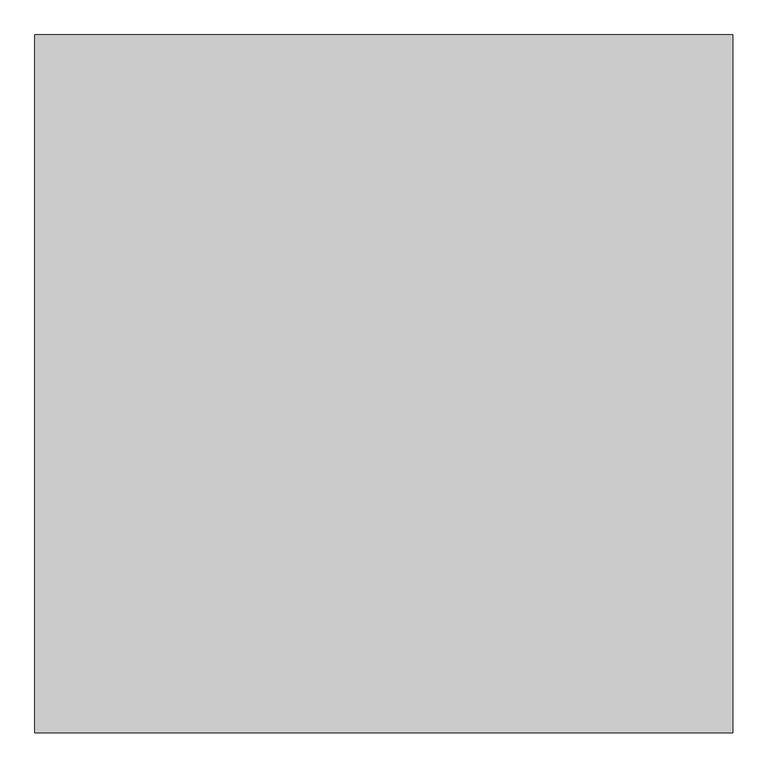
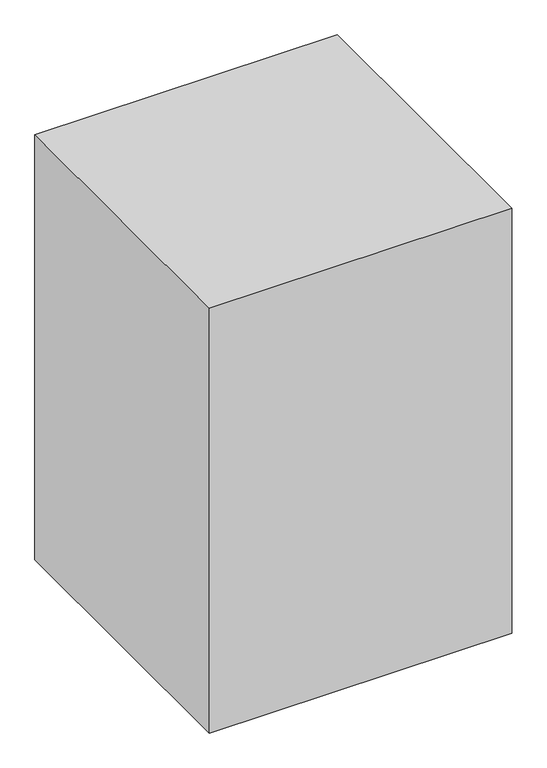
"""IFC4 building model written with IfcOpenShell, lengths in millimetres: proxy geometry, Space Planning Box_hec : Space Planning Box_hec."""

import ifcopenshell
import ifcopenshell.guid

model = None  # the IFC model being written
_history = None  # IfcOwnerHistory: only IFC2X3 demands one
_inside = {}  # id of a spatial element -> (the spatial element, [elements in it])
_under = {}  # id of a project, library or spatial element -> (it, [spatial elements below it])
_declared = {}  # id of a project -> (the project, [libraries it declares])
_typed = {}  # id of a type object -> (the type object, [elements of that type])
_made_of = {}  # id of a material, layer set ... -> (it, [elements and type objects made of it])


def new_model(schema):
    """Start an empty IFC model of exactly this schema.

    Asked for "IFC4X3", IfcOpenShell would pick the latest addendum, in which some entities
    have other attributes; the version numbers below select the first issue.
    IFC2X3 requires an IfcOwnerHistory on every rooted entity: one is made here for all.
    """
    global model, _history
    if schema == "IFC4X3":
        model = ifcopenshell.file(schema_version=(4, 3, 0, 0))
    else:
        model = ifcopenshell.file(schema=schema)
    _inside.clear()
    _under.clear()
    _declared.clear()
    _typed.clear()
    _made_of.clear()
    _history = None
    if model.schema == "IFC2X3":
        org = make("IfcOrganization", Name="unknown")
        user = make(
            "IfcPersonAndOrganization",
            ThePerson=make("IfcPerson", FamilyName="unknown"),
            TheOrganization=org,
        )
        app = make(
            "IfcApplication",
            ApplicationDeveloper=org,
            Version="unknown",
            ApplicationFullName="unknown",
            ApplicationIdentifier="unknown",
        )
        _history = make(
            "IfcOwnerHistory",
            OwningUser=user,
            OwningApplication=app,
            ChangeAction="ADDED",
            CreationDate=0,
        )
    return model


def make(cls, **values):
    """One entity of the class cls with the attributes given. An attribute that is None is left unset."""
    return model.create_entity(
        cls, **{name: value for name, value in values.items() if value is not None}
    )


def rooted(cls, **values):
    """An entity with a GlobalId (a new one), such as an element, a storey or a relation."""
    return make(cls, GlobalId=ifcopenshell.guid.new(), OwnerHistory=_history, **values)


def si_unit(unit_type, name, prefix=None):
    """IfcSIUnit, for example si_unit("LENGTHUNIT", "METRE", prefix="MILLI")."""
    return make("IfcSIUnit", UnitType=unit_type, Prefix=prefix, Name=name)


def assignment(units):
    """IfcUnitAssignment: the units of a project."""
    return None if units is None else make("IfcUnitAssignment", Units=units)


def point(xyz):
    """IfcCartesianPoint."""
    return None if xyz is None else make("IfcCartesianPoint", Coordinates=xyz)


def direction(xyz):
    """IfcDirection."""
    return None if xyz is None else make("IfcDirection", DirectionRatios=xyz)


def frame(location, z_axis=None, x_axis=None):
    """IfcAxis2Placement3D, a coordinate frame: its origin and axes. An axis left out is left unset."""
    return make(
        "IfcAxis2Placement3D",
        Location=point(location),
        Axis=direction(z_axis),
        RefDirection=direction(x_axis),
    )


def origin():
    """The frame at (0, 0, 0) with its axes left unset."""
    return frame((0.0, 0.0, 0.0))


def origin_with_axes():
    """The frame at (0, 0, 0) with the z axis (0, 0, 1) and the x axis (1, 0, 0) written out."""
    return frame((0.0, 0.0, 0.0), z_axis=(0.0, 0.0, 1.0), x_axis=(1.0, 0.0, 0.0))


def place(relative_to, where):
    """IfcLocalPlacement: puts the frame where relative to a parent placement (None: the world)."""
    return make(
        "IfcLocalPlacement", PlacementRelTo=relative_to, RelativePlacement=where
    )


def context(
    kind, dimensions, precision=None, world=None, true_north=None, identifier=None
):
    """IfcGeometricRepresentationContext, for example the 3D "Model" context."""
    return make(
        "IfcGeometricRepresentationContext",
        ContextIdentifier=identifier,
        ContextType=kind,
        CoordinateSpaceDimension=dimensions,
        Precision=precision,
        WorldCoordinateSystem=world,
        TrueNorth=true_north,
    )


def project(units=None, contexts=None):
    """IfcProject with its units and contexts."""
    return rooted(
        "IfcProject",
        Name="project",
        RepresentationContexts=contexts,
        UnitsInContext=assignment(units),
    )


def spatial(cls, under=None, at=None, **own):
    """A site, building, storey or space (cls), placed at a placement, below another one or the project."""
    s = rooted(cls, ObjectPlacement=at, **own)
    if under is not None:
        _under.setdefault(under.id(), (under, []))[1].append(s)
    return s


def polyline(points):
    """IfcPolyline through the points."""
    return make("IfcPolyline", Points=[point(p) for p in points])


def outline(outer, holes=None, kind="AREA"):
    """IfcArbitraryClosedProfileDef: a profile drawn as a closed curve; with holes, ...WithVoids."""
    if holes is None:
        return make("IfcArbitraryClosedProfileDef", ProfileType=kind, OuterCurve=outer)
    return make(
        "IfcArbitraryProfileDefWithVoids",
        ProfileType=kind,
        OuterCurve=outer,
        InnerCurves=holes,
    )


def extrude(swept, where, along, depth):
    """IfcExtrudedAreaSolid: the profile swept, set in the frame where, extruded along a direction by depth."""
    return make(
        "IfcExtrudedAreaSolid",
        SweptArea=swept,
        Position=where,
        ExtrudedDirection=direction(along),
        Depth=depth,
    )


def shape(context_of_items, identifier, shape_type, items):
    """IfcShapeRepresentation: the items that make up one representation, for example the "Body"."""
    return make(
        "IfcShapeRepresentation",
        ContextOfItems=context_of_items,
        RepresentationIdentifier=identifier,
        RepresentationType=shape_type,
        Items=items,
    )


def source(mapping_origin, context_of_items, identifier, shape_type, items):
    """IfcRepresentationMap: a shape defined once, which mapped items show again and again."""
    return make(
        "IfcRepresentationMap",
        MappingOrigin=mapping_origin,
        MappedRepresentation=shape(context_of_items, identifier, shape_type, items),
    )


def transform(
    local_origin,
    x_axis=None,
    y_axis=None,
    z_axis=None,
    scale=None,
    scale2=None,
    scale3=None,
    uniform=True,
):
    """IfcCartesianTransformationOperator3D, or its non-uniform kind. x_axis, y_axis, z_axis: its Axis1, 2, 3."""
    if uniform:
        return make(
            "IfcCartesianTransformationOperator3D",
            Axis1=direction(x_axis),
            Axis2=direction(y_axis),
            LocalOrigin=point(local_origin),
            Scale=scale,
            Axis3=direction(z_axis),
        )
    return make(
        "IfcCartesianTransformationOperator3DnonUniform",
        Axis1=direction(x_axis),
        Axis2=direction(y_axis),
        LocalOrigin=point(local_origin),
        Scale=scale,
        Axis3=direction(z_axis),
        Scale2=scale2,
        Scale3=scale3,
    )


def mapped(mapping_source, mapping_target):
    """IfcMappedItem: shows the shape of a source again, moved by a transform."""
    return make(
        "IfcMappedItem", MappingSource=mapping_source, MappingTarget=mapping_target
    )


def made_of(thing, what):
    """Note that an element or type object is made of a material, layer set ...; save() writes the relation."""
    if what is not None:
        _made_of.setdefault(what.id(), (what, []))[1].append(thing)
    return thing


def element(
    cls,
    number,
    at=None,
    inside=None,
    cuts=None,
    type_object=None,
    material=None,
    context=None,
    identifier="Body",
    shape_type=None,
    held_by="IfcProductDefinitionShape",
    body=None,
    shapes=None,
    **own,
):
    """One element of the class cls, such as IfcWall. Its Tag is "e" and its number.

    at: its placement. inside: the storey or other place that contains it. cuts: it is an
    opening in that element (IfcRelVoidsElement). A single representation is given by context,
    identifier, shape_type and body (its items); several are given by shapes. held_by: the class
    of the entity that holds the representations. save() writes the other relations.
    """
    e = rooted(cls, Tag="e%d" % number, ObjectPlacement=at, **own)
    if body is not None:
        shapes = [shape(context, identifier, shape_type, body)]
    if shapes is not None:
        e.Representation = make(held_by, Representations=shapes)
    if inside is not None:
        _inside.setdefault(inside.id(), (inside, []))[1].append(e)
    if cuts is not None:
        rooted(
            "IfcRelVoidsElement", RelatingBuildingElement=cuts, RelatedOpeningElement=e
        )
    if type_object is not None:
        _typed.setdefault(type_object.id(), (type_object, []))[1].append(e)
    return made_of(e, material)


def aggregate(whole, parts):
    """IfcRelAggregates: a whole, such as a stair, and the parts it consists of."""
    return rooted("IfcRelAggregates", RelatingObject=whole, RelatedObjects=parts)


def save(model, path):
    """Write the relations noted so far, then the file.

    IfcRelAggregates (storeys below a building ...), IfcRelContainedInSpatialStructure (elements
    in a storey), IfcRelDefinesByType, IfcRelAssociatesMaterial and IfcRelDeclares: one each for
    every whole, place, type object, material and project.
    """
    for whole, parts in _under.values():
        aggregate(whole, parts)
    for where, things in _inside.values():
        rooted(
            "IfcRelContainedInSpatialStructure",
            RelatedElements=things,
            RelatingStructure=where,
        )
    for kind, things in _typed.values():
        rooted("IfcRelDefinesByType", RelatedObjects=things, RelatingType=kind)
    for what, things in _made_of.values():
        rooted("IfcRelAssociatesMaterial", RelatedObjects=things, RelatingMaterial=what)
    for by, libraries in _declared.values():
        rooted("IfcRelDeclares", RelatingContext=by, RelatedDefinitions=libraries)
    model.write(path)


def generic_models_412ad42b(model_context):
    return source(origin(), model_context, "Body", "SweptSolid", [
        extrude(outline(polyline([(1750.0, 1750.0), (1750.0, -1750.0), (-1750.0, -1750.0), (-1750.0, 1750.0), (1750.0, 1750.0)])), origin_with_axes(), (0.0, 0.0, 1.0), 5200.0),
    ])


if __name__ == "__main__":
    model = new_model("IFC4")
    model_context = context("Model", 3, world=origin())
    ifc_project = project(units=[si_unit("LENGTHUNIT", "METRE", prefix="MILLI")], contexts=[model_context])
    site = spatial("IfcSite", under=ifc_project)
    building = spatial("IfcBuilding", under=site)
    placement = place(None, origin())
    generic_models_shape = generic_models_412ad42b(model_context)
    element("IfcBuildingElementProxy", 1, Name="Space Planning Box_hec : Space Planning Box_hec", ObjectType="Space Planning Box_hec : Space Planning Box_hec", at=placement, inside=building, context=model_context, shape_type="MappedRepresentation", body=[
        mapped(generic_models_shape, transform((0.0, 0.0, 0.0), x_axis=(1.0, 0.0, 0.0), y_axis=(0.0, 1.0, 0.0), z_axis=(0.0, 0.0, 1.0))),
    ])
    save(model, "model.ifc")

# Revit data of these elements
# Type "Space Planning Box_hec : Space Planning Box_hec"
#   Type Comments = "..."
#   Room Name [instance default] = "?"
#   Interior Finish [instance default] = ""
#   Exterior Finish [instance default] = ""
#   Department [instance default] = ""
#   Assembly Code = "..."
#   ceiling height [instance default] = 0
#   Width [instance default] = 1524 mm
#   Program Area [instance default] = 0.00 m²
#   Length [instance default] = 1524 mm
#   Height [instance default] = 1524 mm
#   Area [instance default] = 2.32258 m²
#   Fill Color [instance default] = Cyan
#   Default Elevation = 0
# Element 1 (IfcBuildingElementProxy, "Space Planning Box_hec : Space Planning Box_hec")
#   Room Name = "Storage"
#   Interior Finish = "IW1..N/A,,WB2..N/A,,FL2..N/A,,CL4..N/A"
#   Exterior Finish = "RF1..N/A,,EW1..N/A"
#   Department = "AR"
#   ceiling height = 2700
#   Width = 3500 mm
#   Program Area = 12.25 m²
#   Length = 3500 mm
#   Height = 5200 mm
#   Area = 12.25 m²
#   Materials on its faces: "Cyan"
# Materials
#   "Cyan": class "Generic", colour RGB 0 255 255, transparency 0.2, Cost = 0
